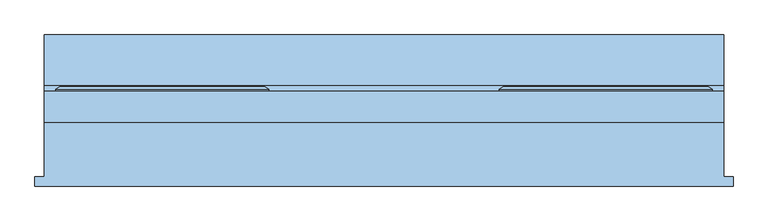
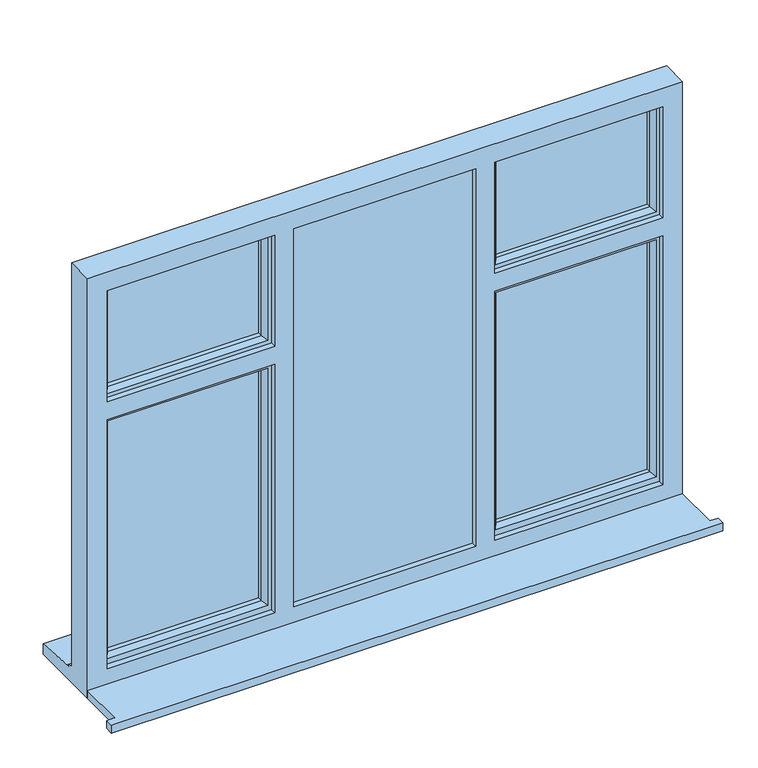
"""IFC4 building model written with IfcOpenShell, lengths in millimetres: window geometry, Window - Triple Casement with Top and Side Sashes : Window - Triple Casement with Top and Side Sashes."""

from ifc_helpers import new_model, si_unit, frame, origin, place, context, project, spatial, polyline, outline, extrude, faceted_brep, source, transform, mapped, element, save


def window_e8f23823(model_context):
    return source(origin(), model_context, "Body", "SolidModel", [
        extrude(outline(polyline([(-1506.6666667, -182.7934322), (-1506.6666667, -157.7934322), (-1481.6666667, -157.7934322), (-1481.6666667, -13.2934322), (328.3333333, -13.2934322), (328.3333333, -157.7934322), (353.3333333, -157.7934322), (353.3333333, -182.7934322), (-1506.6666667, -182.7934322)])), frame((0.0, 0.0, 760.0), z_axis=(0.0, 0.0, 1.0), x_axis=(1.0, 0.0, 0.0)), (0.0, 0.0, 1.0), 25.0),
        extrude(outline(polyline([(823.0, -863.3333333), (823.0, -290.0), (2070.0, -290.0), (2070.0, -863.3333333), (823.0, -863.3333333)]), holes=[polyline([(2060.0, -853.3333333), (2060.0, -300.0), (833.0, -300.0), (833.0, -853.3333333), (2060.0, -853.3333333)])]), frame((0.0, 28.7065678, 0.0), z_axis=(0.0, 1.0, 0.0), x_axis=(0.0, 0.0, 1.0)), (0.0, 0.0, 1.0), 41.0),
        faceted_brep([(-1451.6666667, 69.7065678, 2080.0), (-1451.6666667, 75.4800705, 2080.0), (-1451.6666667, 75.4800705, 1665.0), (-1451.6666667, 69.7065678, 1665.0), (-1441.6666667, 4.7065678, 2070.0), (-1441.6666667, 69.7065678, 2070.0), (-1441.6666667, 69.7065678, 1675.0), (-1441.6666667, 4.7065678, 1675.0), (-1401.6666667, 19.1994677, 2030.0), (-1411.8147044, 4.7065678, 2040.1480377), (-1411.8147044, 4.7065678, 1704.8519623), (-1401.6666667, 19.1994677, 1715.0), (-1401.6666667, 33.7065678, 2030.0), (-1401.6666667, 33.7065678, 1715.0), (-1411.6666667, 57.7065678, 2040.0), (-1411.6666667, 33.7065678, 2040.0), (-1411.6666667, 33.7065678, 1705.0), (-1411.6666667, 57.7065678, 1705.0), (-1401.6666667, 75.4800705, 2030.0), (-1401.6666667, 57.7065678, 2030.0), (-1401.6666667, 57.7065678, 1715.0), (-1401.6666667, 75.4800705, 1715.0), (-1419.1124215, 81.2535732, 2047.4457548), (-1419.1124215, 81.2535732, 1697.5542452), (-1440.882057, 81.2535732, 2069.2153903), (-1440.882057, 81.2535732, 1675.7846097), (-883.3333333, 75.4800705, 1665.0), (-883.3333333, 69.7065678, 1665.0), (-893.3333333, 69.7065678, 1675.0), (-893.3333333, 4.7065678, 1675.0), (-923.1852956, 4.7065678, 1704.8519623), (-933.3333333, 19.1994677, 1715.0), (-933.3333333, 33.7065678, 1715.0), (-923.3333333, 33.7065678, 1705.0), (-923.3333333, 57.7065678, 1705.0), (-933.3333333, 57.7065678, 1715.0), (-933.3333333, 75.4800705, 1715.0), (-915.8875785, 81.2535732, 1697.5542452), (-894.117943, 81.2535732, 1675.7846097), (-883.3333333, 75.4800705, 2080.0), (-883.3333333, 69.7065678, 2080.0), (-893.3333333, 69.7065678, 2070.0), (-893.3333333, 4.7065678, 2070.0), (-923.1852956, 4.7065678, 2040.1480377), (-933.3333333, 19.1994677, 2030.0), (-933.3333333, 33.7065678, 2030.0), (-923.3333333, 33.7065678, 2040.0), (-923.3333333, 57.7065678, 2040.0), (-933.3333333, 57.7065678, 2030.0), (-933.3333333, 75.4800705, 2030.0), (-915.8875785, 81.2535732, 2047.4457548), (-894.117943, 81.2535732, 2069.2153903)], [[[0, 1, 2, 3]], [[4, 5, 6, 7]], [[8, 9, 10, 11]], [[12, 8, 11, 13]], [[14, 15, 16, 17]], [[18, 19, 20, 21]], [[22, 18, 21, 23]], [[1, 24, 25, 2]], [[3, 2, 26, 27]], [[7, 6, 28, 29]], [[11, 10, 30, 31]], [[13, 11, 31, 32]], [[17, 16, 33, 34]], [[21, 20, 35, 36]], [[23, 21, 36, 37]], [[2, 25, 38, 26]], [[27, 26, 39, 40]], [[29, 28, 41, 42]], [[31, 30, 43, 44]], [[32, 31, 44, 45]], [[34, 33, 46, 47]], [[36, 35, 48, 49]], [[37, 36, 49, 50]], [[26, 38, 51, 39]], [[40, 39, 1, 0]], [[3, 27, 40, 0], [5, 41, 28, 6]], [[42, 41, 5, 4]], [[7, 29, 42, 4], [9, 43, 30, 10]], [[44, 43, 9, 8]], [[45, 44, 8, 12]], [[15, 46, 33, 16], [13, 32, 45, 12]], [[47, 46, 15, 14]], [[17, 34, 47, 14], [19, 48, 35, 20]], [[49, 48, 19, 18]], [[50, 49, 18, 22]], [[24, 51, 38, 25], [23, 37, 50, 22]], [[39, 51, 24, 1]]]),
        faceted_brep([(-1451.6666667, 69.7065678, 1655.0), (-1451.6666667, 75.4800705, 1655.0), (-1451.6666667, 75.4800705, 813.0), (-1451.6666667, 69.7065678, 813.0), (-1441.6666667, 4.7065678, 1645.0), (-1441.6666667, 69.7065678, 1645.0), (-1441.6666667, 69.7065678, 823.0), (-1441.6666667, 4.7065678, 823.0), (-1401.6666667, 19.1994677, 1605.0), (-1411.8147044, 4.7065678, 1615.1480377), (-1411.8147044, 4.7065678, 852.8519623), (-1401.6666667, 19.1994677, 863.0), (-1401.6666667, 33.7065678, 1605.0), (-1401.6666667, 33.7065678, 863.0), (-1411.6666667, 57.7065678, 1615.0), (-1411.6666667, 33.7065678, 1615.0), (-1411.6666667, 33.7065678, 853.0), (-1411.6666667, 57.7065678, 853.0), (-1401.6666667, 75.4800705, 1605.0), (-1401.6666667, 57.7065678, 1605.0), (-1401.6666667, 57.7065678, 863.0), (-1401.6666667, 75.4800705, 863.0), (-1419.1124215, 81.2535732, 1622.4457548), (-1419.1124215, 81.2535732, 845.5542452), (-1440.882057, 81.2535732, 1644.2153903), (-1440.882057, 81.2535732, 823.7846097), (-883.3333333, 75.4800705, 813.0), (-883.3333333, 69.7065678, 813.0), (-893.3333333, 69.7065678, 823.0), (-893.3333333, 4.7065678, 823.0), (-923.1852956, 4.7065678, 852.8519623), (-933.3333333, 19.1994677, 863.0), (-933.3333333, 33.7065678, 863.0), (-923.3333333, 33.7065678, 853.0), (-923.3333333, 57.7065678, 853.0), (-933.3333333, 57.7065678, 863.0), (-933.3333333, 75.4800705, 863.0), (-915.8875785, 81.2535732, 845.5542452), (-894.117943, 81.2535732, 823.7846097), (-883.3333333, 75.4800705, 1655.0), (-883.3333333, 69.7065678, 1655.0), (-893.3333333, 69.7065678, 1645.0), (-893.3333333, 4.7065678, 1645.0), (-923.1852956, 4.7065678, 1615.1480377), (-933.3333333, 19.1994677, 1605.0), (-933.3333333, 33.7065678, 1605.0), (-923.3333333, 33.7065678, 1615.0), (-923.3333333, 57.7065678, 1615.0), (-933.3333333, 57.7065678, 1605.0), (-933.3333333, 75.4800705, 1605.0), (-915.8875785, 81.2535732, 1622.4457548), (-894.117943, 81.2535732, 1644.2153903)], [[[0, 1, 2, 3]], [[4, 5, 6, 7]], [[8, 9, 10, 11]], [[12, 8, 11, 13]], [[14, 15, 16, 17]], [[18, 19, 20, 21]], [[22, 18, 21, 23]], [[1, 24, 25, 2]], [[3, 2, 26, 27]], [[7, 6, 28, 29]], [[11, 10, 30, 31]], [[13, 11, 31, 32]], [[17, 16, 33, 34]], [[21, 20, 35, 36]], [[23, 21, 36, 37]], [[2, 25, 38, 26]], [[27, 26, 39, 40]], [[29, 28, 41, 42]], [[31, 30, 43, 44]], [[32, 31, 44, 45]], [[34, 33, 46, 47]], [[36, 35, 48, 49]], [[37, 36, 49, 50]], [[26, 38, 51, 39]], [[40, 39, 1, 0]], [[3, 27, 40, 0], [5, 41, 28, 6]], [[42, 41, 5, 4]], [[7, 29, 42, 4], [9, 43, 30, 10]], [[44, 43, 9, 8]], [[45, 44, 8, 12]], [[15, 46, 33, 16], [13, 32, 45, 12]], [[47, 46, 15, 14]], [[17, 34, 47, 14], [19, 48, 35, 20]], [[49, 48, 19, 18]], [[50, 49, 18, 22]], [[24, 51, 38, 25], [23, 37, 50, 22]], [[39, 51, 24, 1]]]),
        faceted_brep([(-270.0, 69.7065678, 2080.0), (-270.0, 75.4800705, 2080.0), (-270.0, 75.4800705, 1665.0), (-270.0, 69.7065678, 1665.0), (-260.0, 4.7065678, 2070.0), (-260.0, 69.7065678, 2070.0), (-260.0, 69.7065678, 1675.0), (-260.0, 4.7065678, 1675.0), (-220.0, 19.1994677, 2030.0), (-230.1480377, 4.7065678, 2040.1480377), (-230.1480377, 4.7065678, 1704.8519623), (-220.0, 19.1994677, 1715.0), (-220.0, 33.7065678, 2030.0), (-220.0, 33.7065678, 1715.0), (-230.0, 57.7065678, 2040.0), (-230.0, 33.7065678, 2040.0), (-230.0, 33.7065678, 1705.0), (-230.0, 57.7065678, 1705.0), (-220.0, 75.4800705, 2030.0), (-220.0, 57.7065678, 2030.0), (-220.0, 57.7065678, 1715.0), (-220.0, 75.4800705, 1715.0), (-237.4457548, 81.2535732, 2047.4457548), (-237.4457548, 81.2535732, 1697.5542452), (-259.2153903, 81.2535732, 2069.2153903), (-259.2153903, 81.2535732, 1675.7846097), (298.3333333, 75.4800705, 1665.0), (298.3333333, 69.7065678, 1665.0), (288.3333333, 69.7065678, 1675.0), (288.3333333, 4.7065678, 1675.0), (258.4813711, 4.7065678, 1704.8519623), (248.3333333, 19.1994677, 1715.0), (248.3333333, 33.7065678, 1715.0), (258.3333333, 33.7065678, 1705.0), (258.3333333, 57.7065678, 1705.0), (248.3333333, 57.7065678, 1715.0), (248.3333333, 75.4800705, 1715.0), (265.7790881, 81.2535732, 1697.5542452), (287.5487236, 81.2535732, 1675.7846097), (298.3333333, 75.4800705, 2080.0), (298.3333333, 69.7065678, 2080.0), (288.3333333, 69.7065678, 2070.0), (288.3333333, 4.7065678, 2070.0), (258.4813711, 4.7065678, 2040.1480377), (248.3333333, 19.1994677, 2030.0), (248.3333333, 33.7065678, 2030.0), (258.3333333, 33.7065678, 2040.0), (258.3333333, 57.7065678, 2040.0), (248.3333333, 57.7065678, 2030.0), (248.3333333, 75.4800705, 2030.0), (265.7790881, 81.2535732, 2047.4457548), (287.5487236, 81.2535732, 2069.2153903)], [[[0, 1, 2, 3]], [[4, 5, 6, 7]], [[8, 9, 10, 11]], [[12, 8, 11, 13]], [[14, 15, 16, 17]], [[18, 19, 20, 21]], [[22, 18, 21, 23]], [[1, 24, 25, 2]], [[3, 2, 26, 27]], [[7, 6, 28, 29]], [[11, 10, 30, 31]], [[13, 11, 31, 32]], [[17, 16, 33, 34]], [[21, 20, 35, 36]], [[23, 21, 36, 37]], [[2, 25, 38, 26]], [[27, 26, 39, 40]], [[29, 28, 41, 42]], [[31, 30, 43, 44]], [[32, 31, 44, 45]], [[34, 33, 46, 47]], [[36, 35, 48, 49]], [[37, 36, 49, 50]], [[26, 38, 51, 39]], [[40, 39, 1, 0]], [[3, 27, 40, 0], [5, 41, 28, 6]], [[42, 41, 5, 4]], [[7, 29, 42, 4], [9, 43, 30, 10]], [[44, 43, 9, 8]], [[45, 44, 8, 12]], [[15, 46, 33, 16], [13, 32, 45, 12]], [[47, 46, 15, 14]], [[17, 34, 47, 14], [19, 48, 35, 20]], [[49, 48, 19, 18]], [[50, 49, 18, 22]], [[24, 51, 38, 25], [23, 37, 50, 22]], [[39, 51, 24, 1]]]),
        extrude(outline(polyline([(258.3333333, 33.7065678), (-230.1480377, 33.7065678), (-230.1480377, 57.7065678), (258.3333333, 57.7065678), (258.3333333, 33.7065678)])), frame((0.0, 0.0, 852.8519623), z_axis=(0.0, 0.0, 1.0), x_axis=(1.0, 0.0, 0.0)), (0.0, 0.0, 1.0), 762.1480377),
        extrude(outline(polyline([(258.3333333, 33.7065678), (-230.0, 33.7065678), (-230.0, 57.7065678), (258.3333333, 57.7065678), (258.3333333, 33.7065678)])), frame((0.0, 0.0, 1705.0), z_axis=(0.0, 0.0, 1.0), x_axis=(1.0, 0.0, 0.0)), (0.0, 0.0, 1.0), 335.0),
        extrude(outline(polyline([(-923.3333333, 33.7065678), (-1411.6666667, 33.7065678), (-1411.6666667, 57.7065678), (-923.3333333, 57.7065678), (-923.3333333, 33.7065678)])), frame((0.0, 0.0, 1705.0), z_axis=(0.0, 0.0, 1.0), x_axis=(1.0, 0.0, 0.0)), (0.0, 0.0, 1.0), 335.0),
        extrude(outline(polyline([(-923.3333333, 33.7065678), (-1411.6666667, 33.7065678), (-1411.6666667, 57.7065678), (-923.3333333, 57.7065678), (-923.3333333, 33.7065678)])), frame((0.0, 0.0, 853.0), z_axis=(0.0, 0.0, 1.0), x_axis=(1.0, 0.0, 0.0)), (0.0, 0.0, 1.0), 762.0),
        faceted_brep([(-270.0, 69.7065678, 1655.0), (-270.0, 75.4800705, 1655.0), (-270.0, 75.4800705, 813.0), (-270.0, 69.7065678, 813.0), (-260.0, 4.7065678, 1645.0), (-260.0, 69.7065678, 1645.0), (-260.0, 69.7065678, 823.0), (-260.0, 4.7065678, 823.0), (-220.0, 19.1994677, 1605.0), (-230.1480377, 4.7065678, 1615.1480377), (-230.1480377, 4.7065678, 852.8519623), (-220.0, 19.1994677, 863.0), (-220.0, 33.7065678, 1605.0), (-220.0, 33.7065678, 863.0), (-230.0, 57.7065678, 1615.0), (-230.0, 33.7065678, 1615.0), (-230.0, 33.7065678, 853.0), (-230.0, 57.7065678, 853.0), (-220.0, 75.4800705, 1605.0), (-220.0, 57.7065678, 1605.0), (-220.0, 57.7065678, 863.0), (-220.0, 75.4800705, 863.0), (-237.4457548, 81.2535732, 1622.4457548), (-237.4457548, 81.2535732, 845.5542452), (-259.2153903, 81.2535732, 1644.2153903), (-259.2153903, 81.2535732, 823.7846097), (298.3333333, 75.4800705, 813.0), (298.3333333, 69.7065678, 813.0), (288.3333333, 69.7065678, 823.0), (288.3333333, 4.7065678, 823.0), (258.4813711, 4.7065678, 852.8519623), (248.3333333, 19.1994677, 863.0), (248.3333333, 33.7065678, 863.0), (258.3333333, 33.7065678, 853.0), (258.3333333, 57.7065678, 853.0), (248.3333333, 57.7065678, 863.0), (248.3333333, 75.4800705, 863.0), (265.7790881, 81.2535732, 845.5542452), (287.5487236, 81.2535732, 823.7846097), (298.3333333, 75.4800705, 1655.0), (298.3333333, 69.7065678, 1655.0), (288.3333333, 69.7065678, 1645.0), (288.3333333, 4.7065678, 1645.0), (258.4813711, 4.7065678, 1615.1480377), (248.3333333, 19.1994677, 1605.0), (248.3333333, 33.7065678, 1605.0), (258.3333333, 33.7065678, 1615.0), (258.3333333, 57.7065678, 1615.0), (248.3333333, 57.7065678, 1605.0), (248.3333333, 75.4800705, 1605.0), (265.7790881, 81.2535732, 1622.4457548), (287.5487236, 81.2535732, 1644.2153903)], [[[0, 1, 2, 3]], [[4, 5, 6, 7]], [[8, 9, 10, 11]], [[12, 8, 11, 13]], [[14, 15, 16, 17]], [[18, 19, 20, 21]], [[22, 18, 21, 23]], [[1, 24, 25, 2]], [[3, 2, 26, 27]], [[7, 6, 28, 29]], [[11, 10, 30, 31]], [[13, 11, 31, 32]], [[17, 16, 33, 34]], [[21, 20, 35, 36]], [[23, 21, 36, 37]], [[2, 25, 38, 26]], [[27, 26, 39, 40]], [[29, 28, 41, 42]], [[31, 30, 43, 44]], [[32, 31, 44, 45]], [[34, 33, 46, 47]], [[36, 35, 48, 49]], [[37, 36, 49, 50]], [[26, 38, 51, 39]], [[40, 39, 1, 0]], [[3, 27, 40, 0], [5, 41, 28, 6]], [[42, 41, 5, 4]], [[7, 29, 42, 4], [9, 43, 30, 10]], [[44, 43, 9, 8]], [[45, 44, 8, 12]], [[15, 46, 33, 16], [13, 32, 45, 12]], [[47, 46, 15, 14]], [[17, 34, 47, 14], [19, 48, 35, 20]], [[49, 48, 19, 18]], [[50, 49, 18, 22]], [[24, 51, 38, 25], [23, 37, 50, 22]], [[39, 51, 24, 1]]]),
        faceted_brep([(328.3333333, -13.2934322, 2110.0), (-1481.6666667, -13.2934322, 2110.0), (-1481.6666667, -13.2934322, 760.0), (328.3333333, -13.2934322, 760.0), (268.3333333, -13.2934322, 835.0), (-242.0, -13.2934322, 835.0), (-242.0, -13.2934322, 1635.0), (268.3333333, -13.2934322, 1635.0), (-853.3333333, -13.2934322, 2050.0), (-300.0, -13.2934322, 2050.0), (-300.0, -13.2934322, 835.0), (-853.3333333, -13.2934322, 835.0), (-242.0, -13.2934322, 2050.0), (268.3333333, -13.2934322, 2050.0), (268.3333333, -13.2934322, 1693.0), (-242.0, -13.2934322, 1693.0), (-1421.6666667, -13.2934322, 835.0), (-1421.6666667, -13.2934322, 1635.0), (-911.3333333, -13.2934322, 1635.0), (-911.3333333, -13.2934322, 835.0), (-1421.6666667, -13.2934322, 2050.0), (-911.3333333, -13.2934322, 2050.0), (-911.3333333, -13.2934322, 1693.0), (-1421.6666667, -13.2934322, 1693.0), (-1481.6666667, 69.7065678, 2110.0), (-1481.6666667, 69.7065678, 811.0), (-1481.6666667, 84.7065678, 809.68767), (-1481.6666667, 84.7065678, 804.7449676), (-1481.6666667, 219.7065678, 793.8088847), (-1481.6666667, 219.7065678, 760.0), (328.3333333, 69.7065678, 2110.0), (328.3333333, 69.7065678, 811.0), (-260.0, 69.7065678, 823.0), (288.3333333, 69.7065678, 823.0), (288.3333333, 69.7065678, 1645.0), (-260.0, 69.7065678, 1645.0), (288.3333333, 69.7065678, 2070.0), (-260.0, 69.7065678, 2070.0), (-260.0, 69.7065678, 1675.0), (288.3333333, 69.7065678, 1675.0), (-893.3333333, 69.7065678, 823.0), (-893.3333333, 69.7065678, 1645.0), (-1441.6666667, 69.7065678, 1645.0), (-1441.6666667, 69.7065678, 823.0), (-893.3333333, 69.7065678, 2070.0), (-1441.6666667, 69.7065678, 2070.0), (-1441.6666667, 69.7065678, 1675.0), (-893.3333333, 69.7065678, 1675.0), (-853.3333333, 69.7065678, 2070.0), (-853.3333333, 69.7065678, 823.0), (-300.0, 69.7065678, 823.0), (-300.0, 69.7065678, 2070.0), (-1441.6666667, 4.7065678, 2070.0), (-1441.6666667, 4.7065678, 1675.0), (-1441.6666667, 4.7065678, 1645.0), (-1441.6666667, 4.7065678, 823.0), (-893.3333333, 4.7065678, 2070.0), (-893.3333333, 4.7065678, 1675.0), (-911.3333333, 4.7065678, 2050.0), (-1421.6666667, 4.7065678, 2050.0), (-1421.6666667, 4.7065678, 1693.0), (-911.3333333, 4.7065678, 1693.0), (-260.0, 4.7065678, 2070.0), (288.3333333, 4.7065678, 2070.0), (288.3333333, 4.7065678, 1675.0), (-260.0, 4.7065678, 1675.0), (268.3333333, 4.7065678, 2050.0), (-242.0, 4.7065678, 2050.0), (-242.0, 4.7065678, 1693.0), (268.3333333, 4.7065678, 1693.0), (-863.3333333, 4.7065678, 2070.0), (-290.0, 4.7065678, 2070.0), (-290.0, 4.7065678, 823.0), (-863.3333333, 4.7065678, 823.0), (-300.0, 4.7065678, 2050.0), (-853.3333333, 4.7065678, 2050.0), (-853.3333333, 4.7065678, 835.0), (-300.0, 4.7065678, 835.0), (-893.3333333, 4.7065678, 823.0), (-893.3333333, 4.7065678, 1645.0), (-1421.6666667, 4.7065678, 835.0), (-911.3333333, 4.7065678, 835.0), (-911.3333333, 4.7065678, 1635.0), (-1421.6666667, 4.7065678, 1635.0), (288.3333333, 4.7065678, 823.0), (-260.0, 4.7065678, 823.0), (-260.0, 4.7065678, 1645.0), (288.3333333, 4.7065678, 1645.0), (-242.0, 4.7065678, 835.0), (268.3333333, 4.7065678, 835.0), (268.3333333, 4.7065678, 1635.0), (-242.0, 4.7065678, 1635.0), (-853.3333333, 28.7065678, 2070.0), (-300.0, 28.7065678, 2070.0), (-290.0, 28.7065678, 2070.0), (-863.3333333, 28.7065678, 2070.0), (328.3333333, 219.7065678, 760.0), (328.3333333, 219.7065678, 793.8088847), (328.3333333, 84.7065678, 804.7449676), (328.3333333, 84.7065678, 809.68767), (-853.3333333, 28.7065678, 823.0), (-863.3333333, 28.7065678, 823.0), (-290.0, 28.7065678, 823.0), (-300.0, 28.7065678, 823.0)], [[[0, 1, 2, 3], [4, 5, 6, 7], [8, 9, 10, 11], [12, 13, 14, 15], [16, 17, 18, 19], [20, 21, 22, 23]], [[1, 24, 25, 26, 27, 28, 29, 2]], [[24, 30, 31, 25], [32, 33, 34, 35], [36, 37, 38, 39], [40, 41, 42, 43], [44, 45, 46, 47], [48, 49, 50, 51]], [[45, 52, 53, 46]], [[54, 55, 43, 42]], [[52, 56, 57, 53], [58, 59, 60, 61]], [[62, 63, 64, 65], [66, 67, 68, 69]], [[70, 71, 72, 73], [74, 75, 76, 77]], [[78, 55, 54, 79], [80, 81, 82, 83]], [[84, 85, 86, 87], [88, 89, 90, 91]], [[59, 20, 23, 60]], [[16, 80, 83, 17]], [[1, 0, 30, 24]], [[52, 45, 44, 56]], [[36, 63, 62, 37]], [[92, 48, 51, 93, 94, 71, 70, 95]], [[20, 59, 58, 21]], [[66, 13, 12, 67]], [[8, 75, 74, 9]], [[30, 0, 3, 96, 97, 98, 99, 31]], [[63, 36, 39, 64]], [[33, 84, 87, 34]], [[13, 66, 69, 14]], [[89, 4, 7, 90]], [[75, 8, 11, 76]], [[21, 58, 61, 22]], [[81, 19, 18, 82]], [[57, 56, 44, 47]], [[40, 78, 79, 41]], [[49, 48, 92, 100]], [[100, 92, 95, 101]], [[101, 95, 70, 73]], [[94, 102, 72, 71]], [[102, 94, 93, 103]], [[103, 93, 51, 50]], [[37, 62, 65, 38]], [[85, 32, 35, 86]], [[67, 12, 15, 68]], [[5, 88, 91, 6]], [[9, 74, 77, 10]], [[96, 3, 2, 29]], [[97, 96, 29, 28]], [[98, 97, 28, 27]], [[99, 98, 27, 26]], [[31, 99, 26, 25]], [[33, 32, 85, 84]], [[40, 43, 55, 78]], [[50, 49, 100, 101, 73, 72, 102, 103]], [[5, 4, 89, 88]], [[77, 76, 11, 10]], [[81, 80, 16, 19]], [[35, 34, 87, 86]], [[39, 38, 65, 64]], [[15, 14, 69, 68]], [[7, 6, 91, 90]], [[47, 46, 53, 57]], [[42, 41, 79, 54]], [[83, 82, 18, 17]], [[61, 60, 23, 22]]]),
        extrude(outline(polyline([(-863.3333333, 28.7065678), (-290.0, 28.7065678), (-290.0, 4.7065678), (-863.3333333, 4.7065678), (-863.3333333, 28.7065678)])), frame((0.0, 0.0, 823.0), z_axis=(0.0, 0.0, 1.0), x_axis=(1.0, 0.0, 0.0)), (0.0, 0.0, 1.0), 1247.0),
    ])


if __name__ == "__main__":
    model = new_model("IFC4")
    model_context = context("Model", 3, world=origin())
    ifc_project = project(units=[si_unit("LENGTHUNIT", "METRE", prefix="MILLI")], contexts=[model_context])
    site = spatial("IfcSite", under=ifc_project)
    building = spatial("IfcBuilding", under=site)
    placement = place(None, origin())
    window_shape = window_e8f23823(model_context)
    element("IfcWindow", 1, ObjectType="Window - Triple Casement with Top and Side Sashes : Window - Triple Casement with Top and Side Sashes", at=placement, inside=building, context=model_context, shape_type="MappedRepresentation", body=[
        mapped(window_shape, transform((0.0, 0.0, 0.0), x_axis=(1.0, 0.0, 0.0), y_axis=(0.0, 1.0, 0.0), z_axis=(0.0, 0.0, 1.0))),
    ])
    save(model, "model.ifc")

# Revit data of these elements
# Type "Window - Triple Casement with Top and Side Sashes : Window - Triple Casement with Top and Side Sashes"
#   Description = "Triple Casement Window with Opening Sash Vents"
#   Type Mark = "51"
#   Operation = "Userdefined"
#   Manufacturer = "Revit"
#   Keynote = "L10"
#   Wrap Layers (Ext) from Ext = 100 mm
#   Wrap Layers (Int) from Ext = 177.5 mm
#   Window Board Projection = 25 mm
#   Window Board Extension = 25 mm
#   Visual Light Transmittance = 0.9
#   Vent Height = 450 mm
#   Solar Heat Gain Coefficient = 0.78
#   Rough Width = 1810 mm
#   Rough Height = 1350 mm
#   Height = 1350 mm
#   Width = 1810 mm
#   Heat Transfer Coefficient (U) = 3.6886 W/(m²·K)
#   Glazing Thickness = 24 mm
#   FrameOffset - External = 105 mm
#   Frame Depth = 65 mm
#   Default Head Height = 2110 mm
#   Cill Depth = 150 mm
#   Cavity Closer Width = 50 mm
#   Cavity Closer Offset from Ext = 102.5 mm
#   Cavity Closer Depth = 85 mm
#   Vis - Cavity Closers = yes
#   Material Trim = Window Frame
#   Material Glass = Glass
#   Material Frame = Window Frame
#   Construction Type Id = ""
#   Wall Closure = (empty or 0)
#   Analytic Construction = (empty or 0)
# Element 1 (IfcWindow, "Window - Triple Casement with Top and Side Sashes : Window - Triple Casement with Top and Side Sashes")
#   Materials on its faces: "Window Frame", "Glass"
# Materials
#   "Window Frame": class "Miscellaneous", colour RGB 249 249 249, transparency 0, Keynote = "L10"
#   "Glass": class "Glass", colour RGB 0 128 192, transparency 0.9, Description = "Soda Lime Glass", Cost = 0
